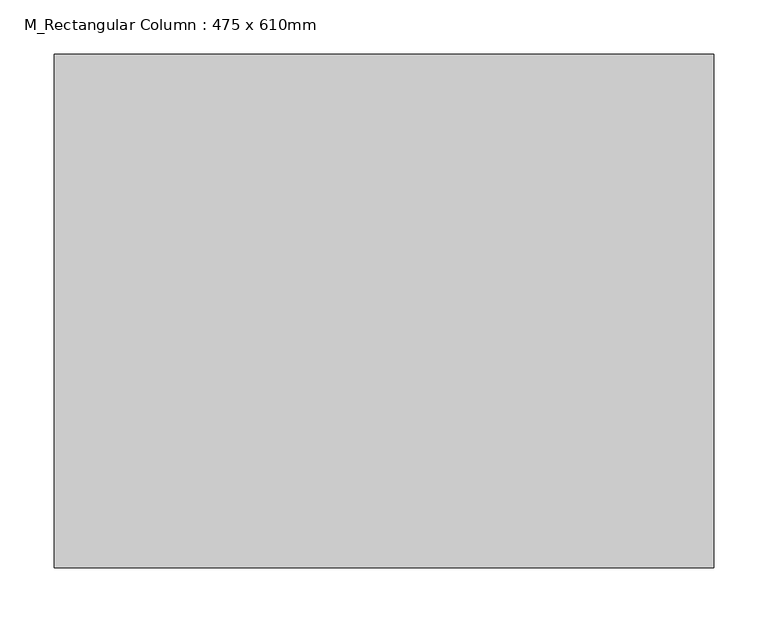
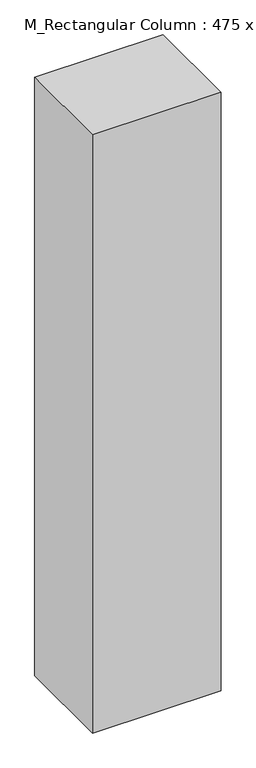
"""IFC4 building model written with IfcOpenShell, lengths in millimetres: column geometry, M_Rectangular Column : 475 x 610mm."""

from ifc_helpers import new_model, si_unit, origin, origin_with_axes, place, context, project, spatial, polyline, outline, extrude, source, transform, mapped, element, save


def m_rectangular_column_475_x_610mm_f11b4c06(model_context):
    return source(origin(), model_context, "Body", "SweptSolid", [
        extrude(outline(polyline([(305.0, 237.5), (305.0, -237.5), (-305.0, -237.5), (-305.0, 237.5), (305.0, 237.5)])), origin_with_axes(), (0.0, 0.0, 1.0), 3000.0),
    ])


if __name__ == "__main__":
    model = new_model("IFC4")
    model_context = context("Model", 3, world=origin())
    ifc_project = project(units=[si_unit("LENGTHUNIT", "METRE", prefix="MILLI")], contexts=[model_context])
    site = spatial("IfcSite", under=ifc_project)
    building = spatial("IfcBuilding", under=site)
    placement = place(None, origin())
    m_rectangular_column_475_x_610mm_shape = m_rectangular_column_475_x_610mm_f11b4c06(model_context)
    element("IfcColumn", 1, ObjectType="M_Rectangular Column : 475 x 610mm", at=placement, inside=building, context=model_context, shape_type="MappedRepresentation", body=[
        mapped(m_rectangular_column_475_x_610mm_shape, transform((0.0, 0.0, 0.0), x_axis=(1.0, 0.0, 0.0), y_axis=(0.0, 1.0, 0.0), z_axis=(0.0, 0.0, 1.0))),
    ])
    save(model, "model.ifc")

# Revit data of these elements
# Type "M_Rectangular Column : 475 x 610mm"
#   Depth = 475 mm
#   Offset Base = 0 mm
#   Offset Top = 0 mm
#   Width = 610 mm
#   Material = Copper
# Element 1 (IfcColumn, "M_Rectangular Column : 475 x 610mm")
#   Materials on its faces: "Copper"
# Materials
#   "Copper": class "Metal", colour RGB 0 0 0, transparency 0, Description = "Copper, matte finish", Cost = 0
